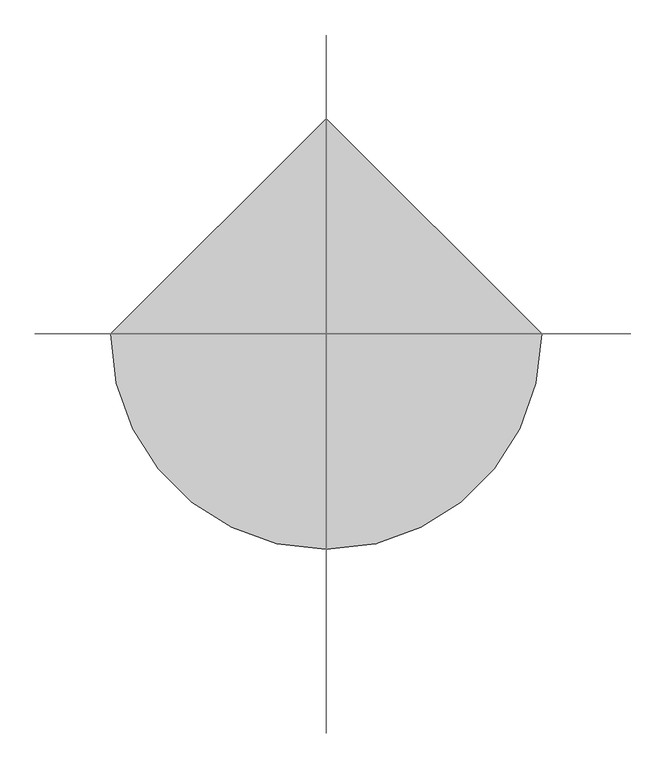
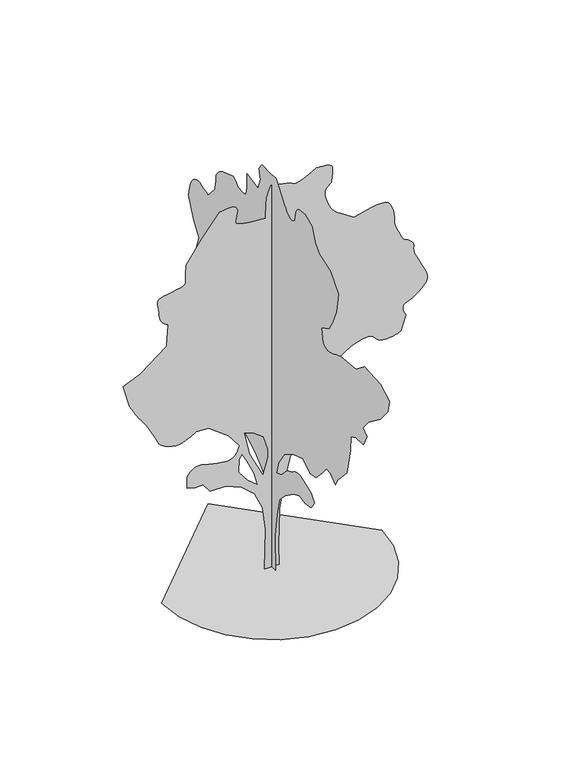
"""IFC4 building model written with IfcOpenShell, lengths in millimetres: geographic element geometry, RPC 木 - 落葉樹 : 桜 - 4.5 メートル."""

from ifc_helpers import new_model, si_unit, origin, place, context, project, spatial, triangles, source, transform, mapped, element, save


def geographic_element_cd2ce576(model_context):
    return source(origin(), model_context, "Body", "Tessellation", [
        triangles([(-0.0027587, 74.5725603, 0.00586), (-0.0027587, -72.0943095, 0.00586), (-0.0027587, -58.7610481, 393.3378007), (-0.0027587, -98.7608322, 653.338028), (-0.0027587, -145.4276149, 853.3381748), (-0.0027587, -252.0952047, 966.670792), (-0.0027587, -412.0928332, 1080.00588), (-0.0027587, -518.7604139, 1126.6709095), (-0.0027587, -625.428031, 1106.6708948), (-0.0027587, -738.7605755, 1126.6709095), (-0.0027587, -798.7606195, 1213.3384392), (-0.0027587, -738.7605755, 1293.3384979), (-0.0027587, -525.4279212, 1366.6710857), (-0.0027587, -506.885412, 1365.1761189), (-0.0027587, -488.5178922, 1363.2711479), (-0.0027587, -470.5003873, 1360.5486397), (-0.0027587, -453.0078504, 1356.6035316), (-0.0027587, -436.2153434, 1351.0261105), (-0.0027587, -420.2953485, 1343.4060814), (-0.0027587, -405.4278331, 1333.3385273), (-0.0027587, -390.5578105, 1322.4935497), (-0.0027587, -374.6402864, 1312.6960373), (-0.0027587, -357.8477795, 1303.7760876), (-0.0027587, -340.3552789, 1295.553479), (-0.0027587, -322.337774, 1287.8585999), (-0.0027587, -303.970236, 1280.5110832), (-0.0027587, -285.4277268, 1273.3385559), (-0.0027587, -185.427399, 1166.6709389), (-0.0027587, -85.4275708, 1126.6709095), (-0.0027587, -125.4276002, 1266.671085), (-0.0027587, -238.7606988, 1433.3386734), (-0.0027587, -398.7603258, 1533.3386742), (-0.0027587, -585.4279653, 1593.3387909), (-0.0027587, -718.7605608, 1506.6712612), (-0.0027587, -825.4281778, 1520.0062031), (-0.0027587, -938.7607224, 1640.0038204), (-0.0027587, -1025.4283247, 1746.6714375), (-0.0027587, -1105.4259127, 1740.0038212), (-0.0027587, -1192.0934423, 1660.0063786), (-0.0027587, -1245.4260155, 1753.3389084), (-0.0027587, -1305.4259869, 1820.0040253), (-0.0027587, -1412.0936039, 1933.3391132), (-0.0027587, -1478.7587208, 2233.3392609), (-0.0027587, -1485.4261917, 2393.3393784), (-0.0027587, -1578.7611923, 2433.336937), (-0.0027587, -1725.426368, 2446.6718788), (-0.0027587, -1785.4264847, 2573.3269386), (-0.0027587, -1712.0938969, 2633.3270554), (-0.0027587, -1812.0938976, 2753.3272888), (-0.0027587, -2038.759132, 2926.6774635), (-0.0027587, -2185.4267784, 3100.0023491), (-0.0027587, -2212.0917206, 3240.0025246), (-0.0027587, -2045.4266029, 3333.3276421), (-0.0027587, -1738.758839, 3346.6776993), (-0.0027587, -1585.4263378, 3226.6774658), (-0.0027587, -1292.0935158, 3193.3274666), (-0.0027587, -1252.2485641, 3177.7025482), (-0.0027587, -1213.3384392, 3162.6025978), (-0.0027587, -1176.2909185, 3148.5525833), (-0.0027587, -1142.0459158, 3136.0774727), (-0.0027587, -1111.5309179, 3125.7025246), (-0.0027587, -1085.6808969, 3117.9524162), (-0.0027587, -1065.4258833, 3113.3274078), (-0.0027587, -1047.2933418, 3113.0774231), (-0.0027587, -1028.108321, 3117.0274727), (-0.0027587, -1009.2758223, 3123.652359), (-0.0027587, -992.1908186, 3131.4524643), (-0.0027587, -978.255768, 3138.9025909), (-0.0027587, -968.8682596, 3144.4775414), (-0.0027587, -965.4257372, 3146.6774071), (-0.0027587, -932.0932514, 3306.6775246), (-0.0027587, -1072.0933542, 3380.0027), (-0.0027587, -1138.7609419, 3486.6778748), (-0.0027587, -1212.093457, 3660.003051), (-0.0027587, -1252.0934864, 3880.0029945), (-0.0027587, -1098.7609125, 4053.3281708), (-0.0027587, -898.760693, 4126.6783447), (-0.0027587, -818.7606342, 4200.0032295), (-0.0027587, -758.7605902, 4360.003347), (-0.0027587, -618.7604874, 4413.3285805), (-0.0027587, -595.9604619, 4413.2285866), (-0.0027587, -573.5129585, 4412.5536278), (-0.0027587, -551.7629416, 4410.70345), (-0.0027587, -531.0629333, 4407.1286682), (-0.0027587, -511.7629123, 4401.17845), (-0.0027587, -494.2128934, 4392.3534073), (-0.0027587, -478.7603846, 4380.0035797), (-0.0027587, -466.2228868, 4364.55336), (-0.0027587, -456.8353784, 4347.0035591), (-0.0027587, -450.0728551, 4327.7035744), (-0.0027587, -445.4078419, 4307.0033844), (-0.0027587, -442.3178415, 4285.2535492), (-0.0027587, -440.2753427, 4262.803466), (-0.0027587, -438.7603552, 4240.0034042), (-0.0027587, -427.2553525, 4227.3033073), (-0.0027587, -415.2803204, 4215.6034401), (-0.0027587, -402.3753304, 4205.9034508), (-0.0027587, -388.070317, 4199.1532814), (-0.0027587, -371.9003011, 4196.3784508), (-0.0027587, -353.3952896, 4198.553318), (-0.0027587, -332.0927745, 4206.6784035), (-0.0027587, -310.9852329, 4218.4782646), (-0.0027587, -293.0277353, 4231.0033722), (-0.0027587, -277.6927156, 4244.1034447), (-0.0027587, -264.4552061, 4257.6784882), (-0.0027587, -252.7927094, 4271.5785118), (-0.0027587, -242.1814384, 4285.7285202), (-0.0027587, -232.0939364, 4300.003521), (-0.0027587, -138.7608616, 4426.6786377), (-0.0027587, -78.7608175, 4500.0035225), (-0.0027587, 21.2393172, 4493.3286392), (-0.0027587, 181.2391372, 4500.0035225), (-0.0027587, 241.2389451, 4420.0034637), (-0.0027587, 214.5724224, 4306.6784042), (-0.0027587, 261.2402133, 4180.0032875), (-0.0027587, 467.9053785, 4220.0034622), (-0.0027587, 467.9053785, 4073.3284035), (-0.0027587, 469.4403866, 4050.6283356), (-0.0027587, 471.6178699, 4028.7032204), (-0.0027587, 475.0778695, 4008.4282951), (-0.0027587, 480.4628969, 3990.6282188), (-0.0027587, 488.4103769, 3976.0532364), (-0.0027587, 499.5679081, 3965.5782944), (-0.0027587, 514.5729152, 3960.0030533), (-0.0027587, 531.7154371, 3957.9281799), (-0.0027587, 548.8579227, 3957.2532211), (-0.0027587, 566.0004447, 3957.7281921), (-0.0027587, 583.1429667, 3959.1531052), (-0.0027587, 600.2854886, 3961.2782661), (-0.0027587, 617.4304813, 3963.853109), (-0.0027587, 634.5730396, 3966.6782272), (-0.0027587, 650.2955538, 3982.2281502), (-0.0027587, 666.0780207, 3996.928125), (-0.0027587, 681.9780676, 4009.8782066), (-0.0027587, 698.0505604, 4020.2031578), (-0.0027587, 714.3580679, 4027.0283226), (-0.0027587, 730.9580721, 4029.4781731), (-0.0027587, 747.9055841, 4026.678344), (-0.0027587, 927.9057163, 3966.6782272), (-0.0027587, 953.4457272, 3949.4781143), (-0.0027587, 977.9358021, 3931.9280228), (-0.0027587, 1000.3257872, 3913.6782646), (-0.0027587, 1019.5682899, 3894.3779892), (-0.0027587, 1034.6108311, 3873.6780899), (-0.0027587, 1044.4058001, 3851.2280067), (-0.0027587, 1047.9058044, 3826.6780518), (-0.0027587, 1048.6833733, 3801.5281334), (-0.0027587, 1050.8608566, 3777.4531494), (-0.0027587, 1054.2033125, 3754.253112), (-0.0027587, 1058.4783422, 3731.7530319), (-0.0027587, 1063.4533293, 3709.7529213), (-0.0027587, 1068.895875, 3688.1280785), (-0.0027587, 1074.570892, 3666.6779343), (-0.0027587, 1201.238451, 3526.6777588), (-0.0027587, 1239.7609543, 3543.5528915), (-0.0027587, 1277.9935043, 3558.9278252), (-0.0027587, 1315.641061, 3571.2779434), (-0.0027587, 1352.4135258, 3579.077758), (-0.0027587, 1388.0210907, 3580.8029434), (-0.0027587, 1422.1711864, 3574.9527191), (-0.0027587, 1454.5710983, 3560.0027596), (-0.0027587, 1482.6961258, 3536.9027161), (-0.0027587, 1504.8736965, 3508.1777252), (-0.0027587, 1522.093721, 3474.8027275), (-0.0027587, 1535.3487259, 3437.7026665), (-0.0027587, 1545.6312378, 3397.8027763), (-0.0027587, 1553.9313126, 3356.02771), (-0.0027587, 1561.2387154, 3313.3277), (-0.0027587, 1474.5711857, 3086.677581), (-0.0027587, 1367.9060394, 2940.0022316), (-0.0027587, 1454.5710983, 2700.0020554), (-0.0027587, 1374.5710396, 2573.3269386), (-0.0027587, 1341.9185268, 2561.8270592), (-0.0027587, 1310.4910847, 2549.851918), (-0.0027587, 1281.5110222, 2536.952124), (-0.0027587, 1256.2035553, 2522.6521248), (-0.0027587, 1235.7959347, 2506.4769493), (-0.0027587, 1221.5109055, 2487.9745903), (-0.0027587, 1214.5709948, 2466.6721115), (-0.0027587, 1212.2984591, 2444.0095413), (-0.0027587, 1211.0734612, 2421.694479), (-0.0027587, 1210.7234825, 2399.6744568), (-0.0027587, 1211.0734612, 2377.8868332), (-0.0027587, 1211.9484804, 2356.2718735), (-0.0027587, 1213.1734783, 2334.7768192), (-0.0027587, 1214.5709948, 2313.3368488), (-0.0027587, 1187.9059799, 2206.6717026), (-0.0027587, 1001.2383041, 2226.6717899), (-0.0027587, 985.728277, 2195.3792233), (-0.0027587, 971.4432478, 2164.9017231), (-0.0027587, 959.6057436, 2136.0591522), (-0.0027587, 951.4432331, 2109.6642517), (-0.0027587, 948.1782434, 2086.536739), (-0.0027587, 951.0357725, 2067.4865936), (-0.0027587, 961.2382748, 2053.3392014), (-0.0027587, 977.7782536, 2041.5990749), (-0.0027587, 998.0507807, 2029.6266953), (-0.0027587, 1020.8883402, 2018.0041489), (-0.0027587, 1045.1258142, 2007.3141037), (-0.0027587, 1069.5958323, 1998.1390823), (-0.0027587, 1093.133349, 1991.0640781), (-0.0027587, 1114.5709213, 1986.6716137), (-0.0027587, 1133.9884134, 1982.8416149), (-0.0027587, 1152.3558969, 1977.2640484), (-0.0027587, 1169.8484339, 1970.2290127), (-0.0027587, 1186.6409409, 1962.0266064), (-0.0027587, 1202.9109507, 1952.9491081), (-0.0027587, 1218.828511, 1943.2890873), (-0.0027587, 1234.5710094, 1933.3391132), (-0.0027587, 1387.9061268, 2013.339172), (-0.0027587, 1431.9861397, 2024.5916828), (-0.0027587, 1474.8436981, 2034.7965832), (-0.0027587, 1515.2512608, 2042.9016117), (-0.0027587, 1551.9862278, 2047.8566872), (-0.0027587, 1583.8238194, 2048.6141991), (-0.0027587, 1609.5388195, 2044.1266823), (-0.0027587, 1627.9038322, 2033.339114), (-0.0027587, 1640.0538174, 2017.6916679), (-0.0027587, 1648.351276, 1999.5965515), (-0.0027587, 1653.4438431, 1979.4615887), (-0.0027587, 1655.9713051, 1957.6915512), (-0.0027587, 1656.5738846, 1934.6990593), (-0.0027587, 1655.8938389, 1910.8890301), (-0.0027587, 1654.5713905, 1886.6714676), (-0.0027587, 1631.6563648, 1862.5889259), (-0.0027587, 1608.3912151, 1839.7339256), (-0.0027587, 1584.4262535, 1819.3239796), (-0.0027587, 1559.4112106, 1802.5889545), (-0.0027587, 1532.9962532, 1790.7539211), (-0.0027587, 1504.833728, 1785.038863), (-0.0027587, 1474.5711857, 1786.6714668), (-0.0027587, 1442.5211071, 1793.7065025), (-0.0027587, 1410.0036152, 1802.1439236), (-0.0027587, 1378.1860806, 1810.1114605), (-0.0027587, 1348.2360191, 1815.7489071), (-0.0027587, 1321.3160053, 1817.1864647), (-0.0027587, 1298.5960258, 1812.5614563), (-0.0027587, 1281.2385098, 1800.0039379), (-0.0027587, 1268.1185257, 1783.8339947), (-0.0027587, 1257.0985588, 1769.4114738), (-0.0027587, 1247.8260143, 1756.448893), (-0.0027587, 1239.9560005, 1744.6513573), (-0.0027587, 1233.1334518, 1733.7264427), (-0.0027587, 1227.0110058, 1723.3863762), (-0.0027587, 1221.2385384, 1713.338879), (-0.0027587, 1243.9585178, 1710.3264175), (-0.0027587, 1265.8635761, 1706.3813095), (-0.0027587, 1286.1360306, 1700.5688736), (-0.0027587, 1303.9584892, 1691.9587887), (-0.0027587, 1318.5160309, 1679.6163734), (-0.0027587, 1328.993589, 1662.608836), (-0.0027587, 1334.5710102, 1640.0038204), (-0.0027587, 1336.8460167, 1613.5137222), (-0.0027587, 1338.0710873, 1585.6212387), (-0.0027587, 1338.4210659, 1556.56371), (-0.0027587, 1338.0710873, 1526.5736801), (-0.0027587, 1337.1961407, 1495.8836929), (-0.0027587, 1335.9710701, 1464.7286179), (-0.0027587, 1334.5710102, 1433.3386734), (-0.0027587, 1300.3260075, 1407.8185741), (-0.0027587, 1266.3110779, 1383.4636654), (-0.0027587, 1232.7634163, 1361.4436432), (-0.0027587, 1199.91593, 1342.9210819), (-0.0027587, 1168.0034157, 1329.0634975), (-0.0027587, 1137.2534031, 1321.0360806), (-0.0027587, 1107.9059212, 1320.0060562), (-0.0027587, 1078.5558958, 1323.638538), (-0.0027587, 1047.808354, 1328.6735504), (-0.0027587, 1015.8932962, 1334.873608), (-0.0027587, 983.0458099, 1342.0060215), (-0.0027587, 949.4982937, 1349.8410084), (-0.0027587, 915.4857622, 1358.1386124), (-0.0027587, 881.238216, 1366.6710857), (-0.0027587, 681.2380692, 1320.0060562), (-0.0027587, 447.9053638, 1200.0059681), (-0.0027587, 314.5727683, 1126.6709095), (-0.0027587, 161.2391225, 1000.0058212), (-0.0027587, 67.9058024, 806.6731453), (-0.0027587, 41.2392842, 533.3379398), (-0.0027587, 67.9058024, 260.0052052), (78.9470616, 0.0002511, 0.0), (-81.0528106, 0.0002511, 0.0), (-67.7195538, 0.0002197, 453.3328669), (-101.05258, 0.0001988, 713.3330578), (-187.7193921, 0.0001884, 899.9981901), (-327.7202579, 0.0001884, 1026.6658218), (-501.0528829, 0.0001779, 1099.9984097), (-667.7180368, 0.0001779, 1099.9984097), (-747.7205664, 0.0001779, 1199.9984831), (-834.3856979, 0.0001779, 1199.9984831), (-921.0532276, 0.0001779, 1219.9984978), (-921.0532276, 0.0001674, 1346.6660568), (-903.7932346, 0.0001674, 1369.3085701), (-885.8332117, 0.0001674, 1390.6686035), (-866.4756723, 0.000157, 1409.4636772), (-845.0181885, 0.000157, 1424.411166), (-820.7606575, 0.000157, 1434.2261192), (-793.0056656, 0.000157, 1437.6286732), (-761.0531101, 0.000157, 1433.3335865), (-723.1130568, 0.000157, 1423.7311203), (-679.5755253, 0.000157, 1412.8461742), (-633.0054754, 0.0001674, 1401.8461189), (-585.970483, 0.0001674, 1391.8936741), (-541.032928, 0.0001674, 1384.1585358), (-500.7603862, 0.0001674, 1379.803569), (-467.71789, 0.0001674, 1379.9986153), (-441.4803563, 0.0001674, 1385.9661289), (-419.4403499, 0.0001674, 1397.5311207), (-400.8978044, 0.000157, 1413.7610893), (-385.1527988, 0.000157, 1433.7212082), (-371.5102813, 0.000157, 1456.4811562), (-359.2652802, 0.000157, 1481.1062519), (-347.7202726, 0.000157, 1506.6661743), (-467.71789, 0.0001465, 1666.6662918), (-687.7180515, 0.000136, 1826.6664093), (-821.0531542, 0.000136, 1833.3314095), (-842.5681927, 0.000136, 1820.5039948), (-864.6081991, 0.000136, 1807.851424), (-887.7006849, 0.000136, 1795.5489773), (-912.3632057, 0.000136, 1783.7688824), (-939.1282871, 0.000136, 1772.6913609), (-968.5158102, 0.000136, 1762.4864605), (-1001.0532864, 0.0001465, 1753.3313507), (-1038.4858126, 0.0001465, 1750.1639568), (-1080.1183731, 0.0001465, 1756.5589153), (-1122.8008696, 0.000136, 1770.6488983), (-1163.385965, 0.000136, 1790.5713741), (-1198.7209448, 0.000136, 1814.4590149), (-1225.6584721, 0.000136, 1840.4465275), (-1241.0509918, 0.000136, 1866.6664387), (-1254.4834568, 0.000136, 1899.3564491), (-1275.8434902, 0.0001256, 1942.8940533), (-1302.4510231, 0.0001256, 1992.6141289), (-1331.6261318, 0.0001256, 2043.8466122), (-1360.6836605, 0.0001256, 2091.9316132), (-1386.9410694, 0.0001151, 2132.204155), (-1407.7185802, 0.0001151, 2159.9992607), (-1425.2510857, 0.0001151, 2182.1367176), (-1443.4812229, 0.0001151, 2208.1242302), (-1462.2962082, 0.0001151, 2237.3167797), (-1481.576136, 0.0001151, 2269.0742889), (-1501.2061878, 0.0001046, 2302.7592968), (-1521.0712543, 0.0001046, 2337.7243137), (-1541.0512848, 0.0001046, 2373.3318787), (-1614.3863434, 9.42e-05, 2626.6771706), (-1421.0511967, 8.37e-05, 2706.6772293), (-1141.0533892, 7.32e-05, 2926.6774635), (-1127.7183746, 5.23e-05, 3166.6526413), (-1147.5834412, 5.23e-05, 3181.0776329), (-1166.6308977, 5.23e-05, 3196.1775833), (-1184.0459684, 5.23e-05, 3212.6774483), (-1199.0109707, 5.23e-05, 3231.2774757), (-1210.7109833, 5.23e-05, 3252.677623), (-1218.3309397, 5.23e-05, 3277.5775566), (-1221.0535206, 5.23e-05, 3306.6525261), (-1223.4635479, 4.19e-05, 3339.402562), (-1228.9034775, 4.19e-05, 3373.552803), (-1234.6960018, 4.19e-05, 3407.2527809), (-1238.155965, 4.19e-05, 3438.6026115), (-1236.6009727, 4.19e-05, 3465.7526985), (-1227.3484852, 4.19e-05, 3486.8278656), (-1207.7184334, 4.19e-05, 3500.0029335), (-1173.335939, 4.19e-05, 3508.2777191), (-1126.1258846, 3.14e-05, 3516.4528015), (-1072.8508661, 3.14e-05, 3525.1778503), (-1020.2758049, 3.14e-05, 3535.2278183), (-975.1632969, 3.14e-05, 3547.2279579), (-944.2782635, 3.14e-05, 3561.9279327), (-934.3857714, 3.14e-05, 3580.0029922), (-936.4657316, 3.14e-05, 3601.7528275), (-937.1457773, 3.14e-05, 3626.6527611), (-936.6582344, 3.14e-05, 3654.1778252), (-935.2407337, 3.14e-05, 3683.7780533), (-933.1232758, 2.09e-05, 3714.9778931), (-930.5382591, 2.09e-05, 3747.2279594), (-927.7182278, 2.09e-05, 3780.0029938), (-761.0531101, 1.05e-05, 4020.00317), (-567.7204705, -1.05e-05, 4260.0033463), (-526.5729095, -1.05e-05, 4266.8535095), (-487.1179049, -1.05e-05, 4272.0284843), (-451.042854, -1.05e-05, 4273.8283745), (-420.0428204, -1.05e-05, 4270.5282852), (-395.80531, -1.05e-05, 4260.4783173), (-380.0228067, -1.05e-05, 4241.9782837), (-374.3852875, 0.0, 4213.3282883), (-377.165314, 0.0, 4181.0532234), (-383.5603088, 0.0, 4152.6032158), (-390.6552973, 0.0, 4127.8032761), (-395.5328339, 0.0, 4106.3534225), (-395.2803057, 0.0, 4088.0533768), (-386.9803036, 0.0, 4072.6781525), (-367.7202873, 0.0, 4060.0033447), (-338.5077536, 0.0, 4049.7280998), (-302.995241, 0.0, 4041.5783066), (-262.2377179, 1.05e-05, 4035.1531174), (-217.282177, 1.05e-05, 4030.1531319), (-169.1771373, 1.05e-05, 4026.1780838), (-118.9730978, 1.05e-05, 4022.9032837), (-67.7195538, 1.05e-05, 4020.00317), (-61.0525507, 0.0, 4200.0032295), (-59.4975493, -1.05e-05, 4225.5284157), (-55.1437952, -1.05e-05, 4250.678334), (-48.4577889, -1.05e-05, 4275.5535599), (-39.9057809, -1.05e-05, 4300.2035088), (-29.954274, -1.05e-05, 4324.6784683), (-19.070066, -1.05e-05, 4349.0284355), (-7.719256, -1.05e-05, 4373.3284058), (37.7812808, -1.05e-05, 4364.7283493), (81.9990646, -1.05e-05, 4356.0285896), (123.6511007, -1.05e-05, 4347.103553), (161.4548797, -1.05e-05, 4337.8035393), (194.127413, -1.05e-05, 4328.053553), (220.3859302, -1.05e-05, 4317.7033127), (238.9474425, -1.05e-05, 4306.6534058), (263.1077047, -1.05e-05, 4303.4283119), (302.4252358, -1.05e-05, 4313.503569), (350.0252918, -1.05e-05, 4332.2035904), (399.0253169, -1.05e-05, 4354.8783691), (442.5428641, -1.05e-05, 4376.8284828), (473.6978665, -2.09e-05, 4393.4286324), (485.6128733, -2.09e-05, 4400.0035217), (495.2154121, -2.09e-05, 4400.2035095), (519.9779268, -2.09e-05, 4399.9285263), (553.8354532, -2.09e-05, 4397.9036499), (590.7254617, -2.09e-05, 4392.8533768), (624.5830244, -1.05e-05, 4383.4783676), (649.3455391, -1.05e-05, 4368.5034096), (658.9480053, -1.05e-05, 4346.6535805), (658.5580582, -1.05e-05, 4321.3283821), (657.4705519, -1.05e-05, 4296.7034317), (655.7980522, -1.05e-05, 4272.6784447), (653.6605373, -1.05e-05, 4249.1034302), (651.1730438, -1.05e-05, 4225.8783943), (648.4505356, 0.0, 4202.8783447), (645.6129908, 0.0, 4180.0032875), (628.6255102, 0.0, 4167.0032089), (612.5730017, 0.0, 4153.2784653), (598.3829885, 0.0, 4138.0032349), (586.992986, 0.0, 4120.4784325), (579.3354592, 0.0, 4099.9282333), (576.3429457, 0.0, 4075.5782661), (578.9479465, 0.0, 4046.6532875), (586.2154535, 1.05e-05, 4014.6032089), (596.2829713, 1.05e-05, 3981.953167), (608.6854846, 1.05e-05, 3949.7530975), (622.9504932, 1.05e-05, 3919.0782257), (638.6155254, 1.05e-05, 3890.9781967), (655.2155296, 1.05e-05, 3866.477948), (672.280549, 2.09e-05, 3846.6529953), (692.3380457, 2.09e-05, 3828.5529373), (717.6455853, 2.09e-05, 3808.6779877), (747.3230616, 2.09e-05, 3787.3531265), (780.5031584, 2.09e-05, 3764.8780449), (816.3031534, 2.09e-05, 3741.5030182), (853.853187, 2.09e-05, 3717.5780251), (892.2807106, 2.09e-05, 3693.3280518), (959.140801, 2.09e-05, 3711.6280975), (1024.3108057, 2.09e-05, 3728.2279564), (1086.098386, 2.09e-05, 3741.4280228), (1142.8159269, 2.09e-05, 3749.5781067), (1192.7659304, 2.09e-05, 3750.9530228), (1234.2634701, 2.09e-05, 3743.8778732), (1265.613446, 2.09e-05, 3726.6530525), (1288.19855, 2.09e-05, 3698.6530174), (1305.0685959, 3.14e-05, 3662.6028923), (1317.0411209, 3.14e-05, 3621.8777618), (1324.9335171, 3.14e-05, 3579.8779999), (1329.5585255, 3.14e-05, 3539.9778191), (1331.7360088, 4.19e-05, 3505.5528854), (1332.2810337, 4.19e-05, 3480.0027008), (1337.451067, 4.19e-05, 3452.7526199), (1350.7835381, 4.19e-05, 3414.6526199), (1369.01353, 4.19e-05, 3371.2026558), (1388.8785965, 5.23e-05, 3327.8526855), (1407.1110592, 5.23e-05, 3290.1026642), (1420.4436756, 5.23e-05, 3263.4275482), (1425.6137089, 5.23e-05, 3253.3275833), (1432.59119, 5.23e-05, 3250.552462), (1450.4136486, 5.23e-05, 3242.5276611), (1474.4187241, 5.23e-05, 3229.7275703), (1499.938678, 5.23e-05, 3212.6024529), (1522.3086788, 5.23e-05, 3191.6275703), (1536.8662205, 5.23e-05, 3167.2776031), (1538.9461807, 6.28e-05, 3140.0025238), (1536.3412525, 6.28e-05, 3112.1024826), (1539.3362732, 6.28e-05, 3085.0273911), (1546.9938, 6.28e-05, 3057.9525902), (1558.3838024, 6.28e-05, 3030.0775475), (1572.5713085, 6.28e-05, 3000.5523148), (1588.6262878, 7.32e-05, 2968.5772316), (1605.6137684, 7.32e-05, 2933.3273483), (1625.0112762, 7.32e-05, 2895.102356), (1646.5088013, 7.32e-05, 2855.2271736), (1666.4888317, 7.32e-05, 2814.5523308), (1681.3363266, 8.37e-05, 2773.8771973), (1687.4413319, 8.37e-05, 2734.0023056), (1681.1813942, 8.37e-05, 2695.7770226), (1658.9462688, 8.37e-05, 2660.0021713), (1628.9963528, 9.42e-05, 2628.8270393), (1601.3762363, 9.42e-05, 2603.2521469), (1575.1563251, 9.42e-05, 2582.3269707), (1549.4036819, 9.42e-05, 2565.1521469), (1523.1837708, 9.42e-05, 2550.7771523), (1495.5661251, 9.42e-05, 2538.2520447), (1465.6137383, 9.42e-05, 2526.6768791), (1440.211219, 9.42e-05, 2513.3021141), (1425.6512066, 9.42e-05, 2496.4220398), (1420.1311947, 9.42e-05, 2476.6369102), (1421.8435902, 0.0001046, 2454.5170395), (1428.976149, 0.0001046, 2430.6494556), (1439.7236034, 0.0001046, 2405.616972), (1452.2811218, 0.0001046, 2379.9993496), (1398.9461506, 0.0001151, 2213.3317612), (1380.1910454, 0.0001151, 2204.8392563), (1360.3261242, 0.0001151, 2196.811694), (1338.2460766, 0.0001151, 2189.7167782), (1312.8435574, 0.0001151, 2184.021777), (1283.0084599, 0.0001151, 2180.194249), (1247.6334389, 0.0001151, 2178.6968113), (1205.6134747, 0.0001151, 2179.9992027), (1167.8684675, 0.0001151, 2188.6467854), (1142.0184465, 0.0001151, 2205.9268353), (1121.9983749, 0.0001151, 2227.4043034), (1101.7459047, 0.0001151, 2248.6467567), (1075.1958538, 0.0001151, 2265.2268494), (1036.2833307, 0.0001151, 2272.7093868), (978.9457695, 0.0001151, 2266.6642616), (912.6507608, 0.0001151, 2247.8318356), (851.8331795, 0.0001151, 2221.3017689), (797.8981722, 0.0001151, 2189.1717533), (752.2405666, 0.0001151, 2153.5467476), (716.2655823, 0.0001151, 2116.5192112), (691.365576, 0.0001256, 2080.1941029), (678.94802, 0.0001256, 2046.6666435), (678.6755075, 0.0001256, 2016.7915775), (688.1980368, 0.0001256, 1989.7166313), (705.8855473, 0.0001256, 1964.9741009), (730.1031097, 0.0001256, 1942.0990437), (759.2181204, 0.000136, 1920.6215755), (791.6006641, 0.000136, 1900.0764633), (825.6131956, 0.000136, 1879.9990551), (845.4582052, 0.000136, 1867.0540604), (864.3707136, 0.000136, 1853.5839523), (881.4156761, 0.000136, 1839.0665245), (895.6632076, 0.000136, 1822.9739021), (906.1781908, 0.000136, 1804.7814079), (912.0281971, 0.000136, 1783.9639286), (912.2807253, 0.000136, 1759.998967), (909.6182425, 0.0001465, 1730.7863605), (907.3057383, 0.0001465, 1695.2763187), (905.28326, 0.0001465, 1654.5187775), (903.4957237, 0.0001465, 1609.5613472), (901.880706, 0.000157, 1561.4562893), (900.3857391, 0.000157, 1511.253685), (898.9457108, 0.000157, 1459.998674), (864.6231691, 0.000157, 1434.5760979), (830.0656855, 0.000157, 1410.9035603), (795.0406431, 0.0001674, 1390.7286289), (759.3156435, 0.0001674, 1375.8010517), (722.6606134, 0.0001674, 1367.8711578), (684.835524, 0.0001674, 1368.686079), (645.6129908, 0.0001674, 1379.9986153), (606.1979911, 0.0001674, 1395.0036587), (567.8304565, 0.0001674, 1406.1611172), (530.3354342, 0.000157, 1414.111068), (493.5429125, 0.000157, 1419.4935883), (457.2753588, 0.000157, 1422.9536968), (421.35782, 0.000157, 1425.1311802), (385.6127998, 0.000157, 1426.6661156), (272.280219, 0.0001674, 1353.3335278), (198.9474132, 0.0001779, 1186.6659393), (125.6138534, 0.0001884, 906.6657337), (85.6140693, 0.0002093, 633.332999), (72.2805581, 0.0002302, 233.3331777), (-94.386072, 8.37e-05, 1079.998395), (-41.0527812, 7.32e-05, 1266.6659981), (-41.0527812, 6.28e-05, 1359.9985279), (-87.7190734, 5.23e-05, 1519.9986454), (-207.7189163, 5.23e-05, 1606.6663204), (-301.052736, 5.23e-05, 1639.9988789), (-241.0526919, 6.28e-05, 1373.3336151), (-154.3856164, 6.28e-05, 993.3332634), (-194.385664, 6.28e-05, 1139.998439), (-267.7202139, 5.23e-05, 1299.9985565), (-321.0527507, 4.19e-05, 1399.9985573), (-354.3852728, 4.19e-05, 1353.3335278), (-361.0527801, 5.23e-05, 1206.665954), (-261.0527066, 6.28e-05, 1079.998395), (-1193.8159389, 0.0, 0.0045206), (-1162.2559467, -273.5427146, 0.0045206), (-1072.3708809, -524.7504189, 0.0045206), (-931.360738, -746.420573, 0.0045206), (-746.420573, -931.360738, 0.0045206), (-524.7504189, -1072.3708809, 0.0045206), (-273.5427146, -1162.2559467, 0.0045206), (5.22e-05, -1193.8159389, 0.0045206), (273.5427146, -1162.2559467, 0.0045206), (524.7504189, -1072.3708809, 0.0045206), (746.420573, -931.360738, 0.0045206), (931.360738, -746.420573, 0.0045206), (1072.3708809, -524.7504189, 0.0045206), (1162.2559467, -273.5427146, 0.0045206), (1193.8159389, 0.0001046, 0.0045206), (-0.0001566, 1193.8159389, 0.0045206)], [[38, 39, 40], [115, 116, 117], [1, 2, 3], [280, 1, 3], [279, 280, 3], [279, 3, 4], [278, 279, 4], [278, 4, 5], [186, 187, 188], [277, 278, 5], [46, 47, 48], [45, 46, 48], [277, 5, 6], [185, 186, 188], [10, 11, 12], [9, 10, 12], [9, 12, 13], [8, 9, 13], [8, 13, 14], [8, 14, 15], [8, 15, 16], [8, 16, 17], [8, 17, 18], [8, 18, 19], [8, 19, 20], [8, 20, 21], [7, 8, 21], [7, 21, 22], [7, 22, 23], [7, 23, 24], [7, 24, 25], [7, 25, 26], [6, 7, 26], [6, 26, 27], [6, 27, 28], [277, 6, 28], [277, 28, 29], [51, 52, 53], [50, 51, 53], [50, 53, 54], [50, 54, 55], [49, 50, 55], [49, 55, 56], [48, 49, 56], [48, 56, 57], [45, 48, 57], [44, 45, 57], [44, 57, 58], [44, 58, 59], [44, 59, 60], [44, 60, 61], [44, 61, 62], [44, 62, 63], [276, 277, 29], [276, 29, 30], [184, 185, 188], [183, 184, 188], [44, 63, 64], [115, 117, 118], [111, 112, 113], [111, 113, 114], [182, 183, 188], [109, 110, 111], [109, 111, 114], [108, 109, 114], [108, 114, 115], [107, 108, 115], [106, 107, 115], [105, 106, 115], [104, 105, 115], [115, 118, 119], [170, 171, 172], [170, 172, 173], [170, 173, 174], [170, 174, 175], [74, 75, 76], [74, 76, 77], [73, 74, 77], [72, 73, 77], [71, 72, 77], [258, 259, 260], [181, 182, 188], [78, 79, 80], [170, 175, 176], [103, 104, 115], [78, 80, 81], [44, 64, 65], [275, 276, 30], [275, 30, 31], [274, 275, 31], [78, 81, 82], [78, 82, 83], [78, 83, 84], [78, 84, 85], [78, 85, 86], [78, 86, 87], [78, 87, 88], [78, 88, 89], [78, 89, 90], [78, 90, 91], [78, 91, 92], [78, 92, 93], [78, 93, 94], [78, 94, 95], [78, 95, 96], [71, 77, 78], [71, 78, 96], [71, 96, 97], [71, 97, 98], [71, 98, 99], [71, 99, 100], [115, 119, 120], [180, 181, 188], [38, 40, 41], [223, 224, 225], [33, 34, 35], [33, 35, 36], [33, 36, 37], [102, 103, 115], [179, 180, 188], [44, 65, 66], [170, 176, 177], [71, 100, 101], [43, 44, 66], [42, 43, 66], [41, 42, 66], [38, 41, 66], [37, 38, 66], [33, 37, 66], [33, 66, 67], [33, 67, 68], [33, 68, 69], [33, 69, 70], [32, 33, 70], [31, 32, 70], [274, 31, 70], [273, 274, 70], [273, 70, 71], [273, 71, 101], [273, 101, 102], [273, 102, 115], [273, 115, 120], [273, 120, 121], [273, 121, 122], [273, 122, 123], [273, 123, 124], [273, 124, 125], [273, 125, 126], [273, 126, 127], [273, 127, 128], [273, 128, 129], [273, 129, 130], [273, 130, 131], [272, 273, 131], [271, 272, 131], [270, 271, 131], [269, 270, 131], [268, 269, 131], [268, 131, 132], [268, 132, 133], [268, 133, 134], [167, 168, 169], [257, 258, 260], [257, 260, 261], [256, 257, 261], [256, 261, 262], [255, 256, 262], [255, 262, 263], [254, 255, 263], [254, 263, 264], [254, 264, 265], [254, 265, 266], [254, 266, 267], [254, 267, 268], [253, 254, 268], [252, 253, 268], [251, 252, 268], [250, 251, 268], [249, 250, 268], [248, 249, 268], [247, 248, 268], [246, 247, 268], [245, 246, 268], [166, 167, 169], [165, 166, 169], [164, 165, 169], [163, 164, 169], [162, 163, 169], [161, 162, 169], [160, 161, 169], [159, 160, 169], [158, 159, 169], [157, 158, 169], [156, 157, 169], [155, 156, 169], [154, 155, 169], [154, 169, 170], [154, 170, 177], [153, 154, 177], [153, 177, 178], [153, 178, 179], [153, 179, 188], [222, 223, 225], [222, 225, 226], [221, 222, 226], [220, 221, 226], [219, 220, 226], [218, 219, 226], [217, 218, 226], [216, 217, 226], [215, 216, 226], [214, 215, 226], [213, 214, 226], [212, 213, 226], [212, 226, 227], [212, 227, 228], [212, 228, 229], [212, 229, 230], [212, 230, 231], [211, 212, 231], [211, 231, 232], [211, 232, 233], [210, 211, 233], [209, 210, 233], [209, 233, 234], [209, 234, 235], [209, 235, 236], [209, 236, 237], [209, 237, 238], [209, 238, 239], [209, 239, 240], [208, 209, 240], [208, 240, 241], [207, 208, 241], [206, 207, 241], [206, 241, 242], [205, 206, 242], [204, 205, 242], [204, 242, 243], [203, 204, 243], [202, 203, 243], [202, 243, 244], [201, 202, 244], [201, 244, 245], [201, 245, 268], [200, 201, 268], [199, 200, 268], [198, 199, 268], [197, 198, 268], [196, 197, 268], [195, 196, 268], [194, 195, 268], [153, 188, 189], [153, 189, 190], [152, 153, 190], [152, 190, 191], [151, 152, 191], [136, 137, 138], [135, 136, 138], [135, 138, 139], [134, 135, 139], [134, 139, 140], [134, 140, 141], [134, 141, 142], [134, 142, 143], [134, 143, 144], [134, 144, 145], [134, 145, 146], [134, 146, 147], [134, 147, 148], [134, 148, 149], [134, 149, 150], [134, 150, 151], [134, 151, 191], [134, 191, 192], [134, 192, 193], [268, 134, 193], [194, 268, 193], [583, 580, 581], [574, 281, 575], [580, 583, 584], [573, 574, 575], [583, 581, 575], [580, 584, 585], [572, 573, 575], [582, 583, 575], [582, 575, 281], [571, 572, 575], [571, 575, 576], [281, 282, 283], [570, 571, 576], [570, 576, 577], [344, 345, 346], [290, 291, 292], [406, 407, 408], [570, 577, 578], [290, 292, 293], [289, 290, 293], [289, 293, 294], [289, 294, 295], [289, 295, 296], [289, 296, 297], [289, 297, 298], [289, 298, 299], [289, 299, 300], [289, 300, 301], [289, 301, 302], [289, 302, 303], [288, 289, 303], [287, 288, 303], [287, 303, 304], [287, 304, 305], [287, 305, 306], [286, 287, 306], [286, 306, 307], [286, 307, 308], [286, 308, 309], [569, 570, 578], [554, 555, 556], [405, 406, 408], [343, 344, 346], [512, 513, 514], [511, 512, 514], [511, 514, 515], [511, 515, 516], [511, 516, 517], [510, 511, 517], [510, 517, 518], [510, 518, 519], [510, 519, 520], [510, 520, 521], [510, 521, 522], [510, 522, 523], [510, 523, 524], [509, 510, 524], [509, 524, 525], [508, 509, 525], [434, 435, 436], [342, 343, 346], [507, 508, 525], [507, 525, 526], [405, 408, 409], [404, 405, 409], [403, 404, 409], [403, 409, 410], [402, 403, 410], [401, 402, 410], [400, 401, 410], [400, 410, 411], [399, 400, 411], [399, 411, 412], [399, 412, 413], [399, 413, 414], [399, 414, 415], [377, 378, 379], [341, 342, 346], [341, 346, 347], [340, 341, 347], [339, 340, 347], [338, 339, 347], [337, 338, 347], [336, 337, 347], [335, 336, 347], [334, 335, 347], [333, 334, 347], [377, 379, 380], [377, 380, 381], [377, 381, 382], [377, 382, 383], [377, 383, 384], [377, 384, 385], [377, 385, 386], [377, 386, 387], [377, 387, 388], [377, 388, 389], [377, 389, 390], [377, 390, 391], [376, 377, 391], [376, 391, 392], [375, 376, 392], [374, 375, 392], [373, 374, 392], [372, 373, 392], [372, 392, 393], [371, 372, 393], [370, 371, 393], [369, 370, 393], [369, 393, 394], [369, 394, 395], [369, 395, 396], [332, 333, 347], [369, 396, 397], [426, 427, 428], [426, 428, 429], [425, 426, 429], [425, 429, 430], [424, 425, 430], [424, 430, 431], [423, 424, 431], [423, 431, 432], [422, 423, 432], [422, 432, 433], [421, 422, 433], [420, 421, 433], [419, 420, 433], [418, 419, 433], [418, 433, 434], [418, 434, 436], [418, 436, 437], [418, 437, 438], [418, 438, 439], [417, 418, 439], [417, 439, 440], [416, 417, 440], [416, 440, 441], [415, 416, 441], [399, 415, 441], [399, 441, 442], [399, 442, 443], [399, 443, 444], [399, 444, 445], [399, 445, 446], [399, 446, 447], [399, 447, 448], [399, 448, 449], [369, 397, 398], [331, 332, 347], [368, 369, 398], [360, 361, 362], [359, 360, 362], [359, 362, 363], [358, 359, 363], [358, 363, 364], [357, 358, 364], [357, 364, 365], [356, 357, 365], [355, 356, 365], [355, 365, 366], [354, 355, 366], [353, 354, 366], [352, 353, 366], [351, 352, 366], [350, 351, 366], [349, 350, 366], [348, 349, 366], [348, 366, 367], [348, 367, 368], [348, 368, 398], [347, 348, 398], [347, 398, 399], [347, 399, 449], [347, 449, 450], [347, 450, 451], [347, 451, 452], [331, 347, 452], [331, 452, 453], [331, 453, 454], [331, 454, 455], [331, 455, 456], [330, 331, 456], [329, 330, 456], [328, 329, 456], [327, 328, 456], [326, 327, 456], [325, 326, 456], [324, 325, 456], [323, 324, 456], [322, 323, 456], [321, 322, 456], [320, 321, 456], [319, 320, 456], [318, 319, 456], [317, 318, 456], [316, 317, 456], [315, 316, 456], [314, 315, 456], [314, 456, 457], [314, 457, 458], [314, 458, 459], [314, 459, 460], [314, 460, 461], [314, 461, 462], [314, 462, 463], [314, 463, 464], [314, 464, 465], [314, 465, 466], [314, 466, 467], [314, 467, 468], [314, 468, 469], [314, 469, 470], [314, 470, 471], [314, 471, 472], [314, 472, 473], [314, 473, 474], [314, 474, 475], [314, 475, 476], [314, 476, 477], [314, 477, 478], [314, 478, 479], [314, 479, 480], [314, 480, 481], [314, 481, 482], [314, 482, 483], [314, 483, 484], [314, 484, 485], [314, 485, 486], [314, 486, 487], [314, 487, 488], [314, 488, 489], [314, 489, 490], [314, 490, 491], [314, 491, 492], [314, 492, 493], [314, 493, 494], [314, 494, 495], [314, 495, 496], [314, 496, 497], [314, 497, 498], [314, 498, 499], [314, 499, 500], [314, 500, 501], [314, 501, 502], [580, 585, 586], [554, 556, 557], [553, 554, 557], [553, 557, 558], [553, 558, 559], [553, 559, 560], [553, 560, 561], [553, 561, 562], [553, 562, 563], [552, 553, 563], [552, 563, 564], [551, 552, 564], [550, 551, 564], [550, 564, 565], [549, 550, 565], [549, 565, 566], [548, 549, 566], [547, 548, 566], [546, 547, 566], [545, 546, 566], [544, 545, 566], [543, 544, 566], [542, 543, 566], [541, 542, 566], [540, 541, 566], [539, 540, 566], [538, 539, 566], [538, 566, 567], [537, 538, 567], [537, 567, 568], [537, 568, 569], [537, 569, 578], [536, 537, 578], [535, 536, 578], [535, 578, 579], [534, 535, 579], [534, 579, 580], [533, 534, 580], [532, 533, 580], [507, 526, 527], [506, 507, 527], [531, 532, 580], [506, 527, 528], [530, 531, 580], [281, 283, 284], [582, 281, 284], [582, 284, 285], [582, 285, 286], [588, 582, 286], [587, 588, 286], [587, 286, 309], [586, 587, 309], [586, 309, 310], [586, 310, 311], [586, 311, 312], [586, 312, 313], [580, 586, 313], [580, 313, 314], [530, 580, 314], [529, 530, 314], [502, 503, 504], [502, 504, 505], [314, 502, 505], [529, 314, 505], [529, 505, 506], [529, 506, 528], [603, 604, 589], [602, 603, 589], [602, 589, 590], [601, 602, 590], [601, 590, 591], [601, 591, 592], [600, 601, 592], [599, 600, 592], [599, 592, 593], [599, 593, 594], [599, 594, 595], [599, 595, 596], [599, 596, 597], [599, 597, 598]], closed=False),
    ])


if __name__ == "__main__":
    model = new_model("IFC4")
    model_context = context("Model", 3, world=origin())
    ifc_project = project(units=[si_unit("LENGTHUNIT", "METRE", prefix="MILLI")], contexts=[model_context])
    site = spatial("IfcSite", under=ifc_project)
    building = spatial("IfcBuilding", under=site)
    placement = place(None, origin())
    geographic_element_shape = geographic_element_cd2ce576(model_context)
    element("IfcGeographicElement", 1, ObjectType="RPC 木 - 落葉樹 : 桜 - 4.5 メートル", at=placement, inside=building, context=model_context, shape_type="MappedRepresentation", body=[
        mapped(geographic_element_shape, transform((0.0, 0.0, 0.0), x_axis=(1.0, 0.0, 0.0), y_axis=(0.0, 1.0, 0.0), z_axis=(0.0, 0.0, 1.0))),
    ])
    save(model, "model.ifc")

# Revit data of these elements
# Type "RPC 木 - 落葉樹 : 桜 - 4.5 メートル"
#   built-in parameter 1005198 = "{2, 15},{39, RPC-16-FXGW-2MQ0-PN7K-A000-ST1L-LVER-AU},{1, 0},{1, 0},{2, 35},{1, 8},{5, Color},{1, 0},{1, 0},{3, 0.8},{3, 0.8},{3, 0.8},{1, 8},{7, BBoxMin},{1, 0},{1, 0},{1, 0},{1, 0},{1, 0},{1, 8},{7, BBoxMax},{1, 0},{1, 0},{1, 0},{1, 0},{1, 0},{2, 11},{9, RPCTypeId},{1, 0},{1, 0},{39, RPC-16-FXGW-2MQ0-PN7K-A000-ST1L-LVER-AU},{1, 6},{14, RPCPlantHeight},{1, 0},{1, 0},{7, 14.7638},{2, 11},{7, keyword},{1, 0},{1, 0},{207, :Geometry:RPC:Japanese Flowering Cherry:Prunus serrulata Lindl:A landscape tree:valued for its abundant showy flowers; native to China and Japan.  Hardy only in the mildest parts of Canada and farther south.},{2, 11},{8, category},{1, 0},{1, 0},{16, :Trees [General]},{2, 11},{12, LocalizedUID},{1, 0},{1, 0},{25, Japanese Flowering Cherry},{2, 14},{6, Height},{1, 0},{1, 0},{7, 14.7638},{1, 2},{16, Cast Reflections},{1, 0},{1, 0},{1, 0},{1, 2},{12, Cast Shadows},{1, 0},{1, 0},{1, 1},{1, 2},{9, Lock View},{1, 0},{1, 0},{1, 0},{1, 4},{5, ViewC},{1, 0},{1, 0},{1, 0},{2, 11},{20, AdvancedUIDefinition},{1, 0},{1, 0},{0, },{2, 11},{10, AssetLibID},{1, 0},{1, 0},{36, 4D3F6E72-3F99-4203-98E9-AF80B3C7A7A4},{2, 11},{10, BaseSchema},{1, 0},{1, 0},{9, RPCSchema},{2, 11},{12, ExchangeGUID},{1, 0},{1, 0},{0, },{1, 2},{6, Hidden},{1, 0},{1, 0},{1, 0},{1, 4},{11, RPCCategory},{1, 0},{1, 0},{1, 0},{2, 11},{8, RPCImage},{1, 0},{1, 0},{0, },{1, 4},{13, SchemaVersion},{1, 0},{1, 0},{1, 4},{2, 11},{12, UIDefinition},{1, 0},{1, 0},{0, },{2, 11},{6, UIName},{1, 0},{1, 0},{39, RPC-16-FXGW-2MQ0-PN7K-A000-ST1L-LVER-AU},{2, 11},{11, VersionGUID},{1, 0},{1, 0},{9, RPCSchema},{2, 11},{9, assettype},{1, 0},{1, 0},{11, RPCGeometry},{2, 11},{11, description},{1, 0},{1, 0},{0, },{2, 11},{9, localname},{1, 0},{1, 0},{3, RPC},{2, 11},{9, localtype},{1, 0},{1, 0},{3, RPC},{1, 4},{8, revision},{1, 0},{1, 0},{1, 1},{2, 11},{9, thumbnail},{1, 0},{1, 0},{0, },{1, 4},{7, version},{1, 0},{1, 0},{1, 1},{1, 2},{20, RPC_Cast Reflections},{1, 0},{1, 0},{1, 1},{1, 2},{16, RPC_Cast Shadows},{1, 0},{1, 0},{1, 1},{1, 2},{13, RPC_Lock View},{1, 0},{1, 0},{1, 0},{1, 4},{9, RPC_ViewC},{1, 0},{1, 0},{1, 0},{21, assetlibrary_base.fbx},{1, 5},"
#   built-in parameter 1005195 = "RPC-16-FXGW-2MQ0-PN7K-A000-ST1L-LVER-AU"
#   Type Comments = "桜"
#   Height = 4500 mm
#   Default Elevation = 0
